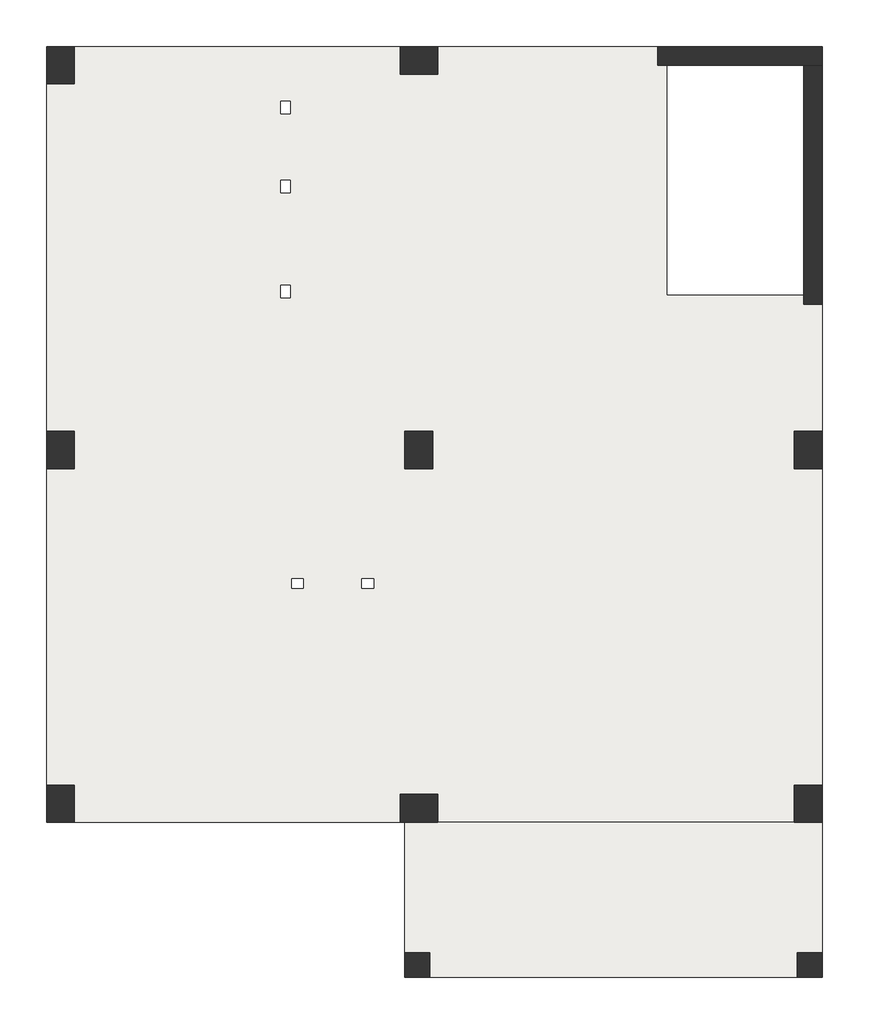
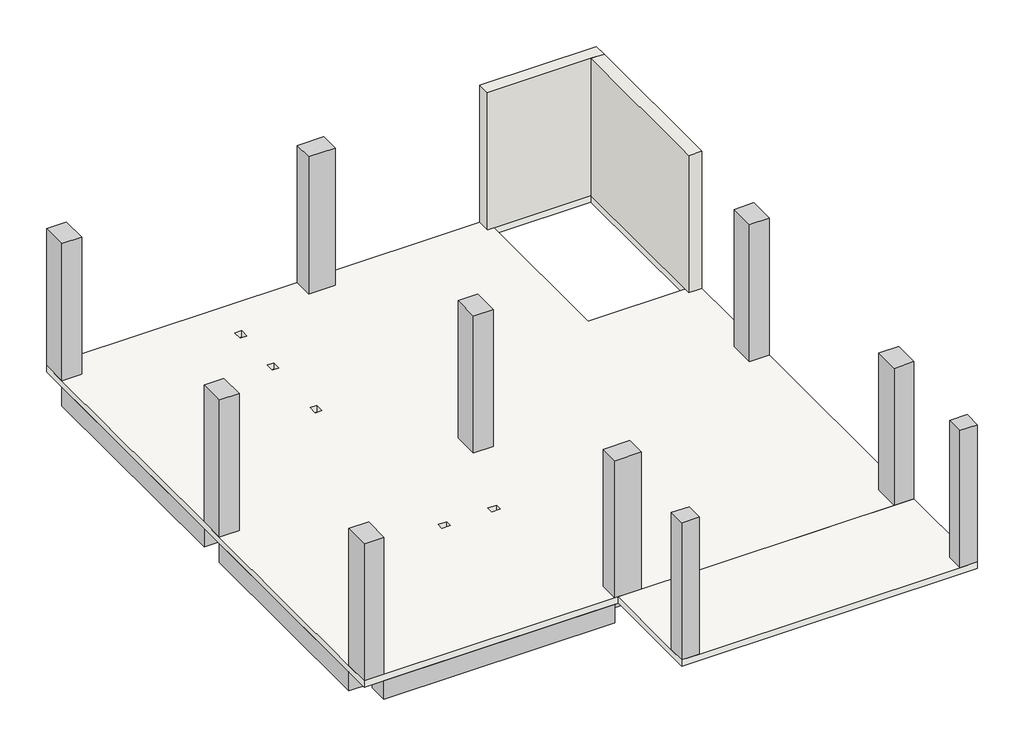
# One storey: 12 beams, 10 columns, 2 slabs, 2 walls.
"""IFC4 building model written with IfcOpenShell, lengths in millimetres."""

from ifc_helpers import new_model, si_unit, frame, origin, place, context, project, spatial, polyline, outline, extrude, faceted_brep, element, save

model = new_model("IFC4")

# Units and contexts
model_context = context("Model", 3, world=origin())
ifc_project = project(units=[si_unit("LENGTHUNIT", "METRE", prefix="MILLI")], contexts=[model_context])

# Site, building, storey
site = spatial("IfcSite", under=ifc_project)
building = spatial("IfcBuilding", under=site)
storey = spatial("IfcBuildingStorey", under=building, Name="01-Birinci Kat", Elevation=97280.0)

# Beams
placement = place(None, origin())
element("IfcBeam", 1, ObjectType="M_Concrete-Rectangular Beam : 45x60cm Kiriş", at=placement, inside=storey, context=model_context, shape_type="SweptSolid", body=[
    extrude(outline(polyline([(5700.0, 14550.0), (450.0, 14550.0), (450.0, 15000.0), (5700.0, 15000.0), (5700.0, 14550.0)])), frame((0.0, 0.0, 96680.0), z_axis=(0.0, 0.0, 1.0), x_axis=(1.0, 0.0, 0.0)), (0.0, 0.0, 1.0), 450.0),
])
element("IfcBeam", 2, ObjectType="M_Concrete-Rectangular Beam : 45x60cm Kiriş", at=placement, inside=storey, context=model_context, shape_type="SweptSolid", body=[
    extrude(outline(polyline([(0.0, 3100.0), (0.0, 8200.0), (450.0, 8200.0), (450.0, 3100.0), (0.0, 3100.0)])), frame((0.0, 0.0, 96680.0), z_axis=(0.0, 0.0, 1.0), x_axis=(1.0, 0.0, 0.0)), (0.0, 0.0, 1.0), 450.0),
])
element("IfcBeam", 3, ObjectType="M_Concrete-Rectangular Beam : 45x60cm Kiriş", at=placement, inside=storey, context=model_context, shape_type="SweptSolid", body=[
    extrude(outline(polyline([(5700.0, 2500.0), (450.0, 2500.0), (450.0, 2950.0), (5700.0, 2950.0), (5700.0, 2500.0)])), frame((0.0, 0.0, 96680.0), z_axis=(0.0, 0.0, 1.0), x_axis=(1.0, 0.0, 0.0)), (0.0, 0.0, 1.0), 450.0),
])
element("IfcBeam", 4, ObjectType="M_Concrete-Rectangular Beam : 45x60cm Kiriş", at=placement, inside=storey, context=model_context, shape_type="SweptSolid", body=[
    extrude(outline(polyline([(12050.0, 2500.0), (6300.0, 2500.0), (6300.0, 2950.0), (12050.0, 2950.0), (12050.0, 2500.0)])), frame((0.0, 0.0, 96680.0), z_axis=(0.0, 0.0, 1.0), x_axis=(1.0, 0.0, 0.0)), (0.0, 0.0, 1.0), 450.0),
])
element("IfcBeam", 5, ObjectType="M_Concrete-Rectangular Beam : 45x60cm Kiriş", at=placement, inside=storey, context=model_context, shape_type="SweptSolid", body=[
    extrude(outline(polyline([(12500.0, 8200.0), (12500.0, 3100.0), (12050.0, 3100.0), (12050.0, 8200.0), (12500.0, 8200.0)])), frame((0.0, 0.0, 96680.0), z_axis=(0.0, 0.0, 1.0), x_axis=(1.0, 0.0, 0.0)), (0.0, 0.0, 1.0), 450.0),
])
element("IfcBeam", 6, ObjectType="M_Concrete-Rectangular Beam : 45x60cm Kiriş", at=placement, inside=storey, context=model_context, shape_type="SweptSolid", body=[
    extrude(outline(polyline([(0.0, 8800.0), (0.0, 14400.0), (450.0, 14400.0), (450.0, 8800.0), (0.0, 8800.0)])), frame((0.0, 0.0, 96680.0), z_axis=(0.0, 0.0, 1.0), x_axis=(1.0, 0.0, 0.0)), (0.0, 0.0, 1.0), 450.0),
])
element("IfcBeam", 7, ObjectType="M_Concrete-Rectangular Beam : 45x60cm Kiriş", at=placement, inside=storey, context=model_context, shape_type="SweptSolid", body=[
    extrude(outline(polyline([(5775.0, 8800.0), (5775.0, 14550.0), (6225.0, 14550.0), (6225.0, 8800.0), (5775.0, 8800.0)])), frame((0.0, 0.0, 96680.0), z_axis=(0.0, 0.0, 1.0), x_axis=(1.0, 0.0, 0.0)), (0.0, 0.0, 1.0), 450.0),
])
element("IfcBeam", 8, ObjectType="M_Concrete-Rectangular Beam : 30x60cm Kiriş", at=placement, inside=storey, context=model_context, shape_type="SweptSolid", body=[
    extrude(outline(polyline([(9850.0, 15000.0), (9850.0, 14700.0), (6300.0, 14700.0), (6300.0, 15000.0), (9850.0, 15000.0)])), frame((0.0, 0.0, 96680.0), z_axis=(0.0, 0.0, 1.0), x_axis=(1.0, 0.0, 0.0)), (0.0, 0.0, 1.0), 450.0),
])
element("IfcBeam", 9, ObjectType="M_Concrete-Rectangular Beam : 30x60cm Kiriş", at=placement, inside=storey, context=model_context, shape_type="SweptSolid", body=[
    extrude(outline(polyline([(12200.0, 10850.0), (12500.0, 10850.0), (12500.0, 8800.0), (12200.0, 8800.0), (12200.0, 10850.0)])), frame((0.0, 0.0, 96680.0), z_axis=(0.0, 0.0, 1.0), x_axis=(1.0, 0.0, 0.0)), (0.0, 0.0, 1.0), 450.0),
])
element("IfcBeam", 10, ObjectType="M_Concrete-Rectangular Beam : 45x60cm Kiriş", at=placement, inside=storey, context=model_context, shape_type="SweptSolid", body=[
    extrude(outline(polyline([(5775.0, 2950.0), (5775.0, 8200.0), (6225.0, 8200.0), (6225.0, 2950.0), (5775.0, 2950.0)])), frame((0.0, 0.0, 96680.0), z_axis=(0.0, 0.0, 1.0), x_axis=(1.0, 0.0, 0.0)), (0.0, 0.0, 1.0), 450.0),
])
element("IfcBeam", 11, ObjectType="M_Concrete-Rectangular Beam : 45x60cm Kiriş", at=placement, inside=storey, context=model_context, shape_type="SweptSolid", body=[
    extrude(outline(polyline([(5775.0, 8275.0), (450.0, 8275.0), (450.0, 8725.0), (5775.0, 8725.0), (5775.0, 8275.0)])), frame((0.0, 0.0, 96680.0), z_axis=(0.0, 0.0, 1.0), x_axis=(1.0, 0.0, 0.0)), (0.0, 0.0, 1.0), 450.0),
])
element("IfcBeam", 12, ObjectType="M_Concrete-Rectangular Beam : 45x60cm Kiriş", at=placement, inside=storey, context=model_context, shape_type="SweptSolid", body=[
    extrude(outline(polyline([(12050.0, 8275.0), (6225.0, 8275.0), (6225.0, 8725.0), (12050.0, 8725.0), (12050.0, 8275.0)])), frame((0.0, 0.0, 96680.0), z_axis=(0.0, 0.0, 1.0), x_axis=(1.0, 0.0, 0.0)), (0.0, 0.0, 1.0), 450.0),
])

# Columns
element("IfcColumn", 13, ObjectType="M_Concrete-Rectangular-Column : 45x60cm Kolon", at=placement, inside=storey, context=model_context, shape_type="SweptSolid", body=[
    extrude(outline(polyline([(450.0, 15000.0), (450.0, 14400.0), (0.0, 14400.0), (0.0, 15000.0), (450.0, 15000.0)])), frame((0.0, 0.0, 97280.0), z_axis=(0.0, 0.0, 1.0), x_axis=(1.0, 0.0, 0.0)), (0.0, 0.0, 1.0), 3300.0),
])
element("IfcColumn", 14, ObjectType="M_Concrete-Rectangular-Column : 45x60cm Kolon", at=placement, inside=storey, context=model_context, shape_type="SweptSolid", body=[
    extrude(outline(polyline([(450.0, 8800.0), (450.0, 8200.0), (0.0, 8200.0), (0.0, 8800.0), (450.0, 8800.0)])), frame((0.0, 0.0, 97280.0), z_axis=(0.0, 0.0, 1.0), x_axis=(1.0, 0.0, 0.0)), (0.0, 0.0, 1.0), 3300.0),
])
element("IfcColumn", 15, ObjectType="M_Concrete-Rectangular-Column : 45x60cm Kolon", at=placement, inside=storey, context=model_context, shape_type="SweptSolid", body=[
    extrude(outline(polyline([(450.0, 3100.0), (450.0, 2500.0), (0.0, 2500.0), (0.0, 3100.0), (450.0, 3100.0)])), frame((0.0, 0.0, 97280.0), z_axis=(0.0, 0.0, 1.0), x_axis=(1.0, 0.0, 0.0)), (0.0, 0.0, 1.0), 3300.0),
])
element("IfcColumn", 16, ObjectType="M_Concrete-Rectangular-Column : 45x60cm Kolon", at=placement, inside=storey, context=model_context, shape_type="SweptSolid", body=[
    extrude(outline(polyline([(6225.0, 8800.0), (6225.0, 8200.0), (5775.0, 8200.0), (5775.0, 8800.0), (6225.0, 8800.0)])), frame((0.0, 0.0, 97280.0), z_axis=(0.0, 0.0, 1.0), x_axis=(1.0, 0.0, 0.0)), (0.0, 0.0, 1.0), 3300.0),
])
element("IfcColumn", 17, ObjectType="M_Concrete-Rectangular-Column : 45x60cm Kolon", at=placement, inside=storey, context=model_context, shape_type="SweptSolid", body=[
    extrude(outline(polyline([(12500.0, 8800.0), (12500.0, 8200.0), (12050.0, 8200.0), (12050.0, 8800.0), (12500.0, 8800.0)])), frame((0.0, 0.0, 97280.0), z_axis=(0.0, 0.0, 1.0), x_axis=(1.0, 0.0, 0.0)), (0.0, 0.0, 1.0), 3300.0),
])
element("IfcColumn", 18, ObjectType="M_Concrete-Rectangular-Column : 45x60cm Kolon", at=placement, inside=storey, context=model_context, shape_type="SweptSolid", body=[
    extrude(outline(polyline([(12500.0, 3100.0), (12500.0, 2500.0), (12050.0, 2500.0), (12050.0, 3100.0), (12500.0, 3100.0)])), frame((0.0, 0.0, 97280.0), z_axis=(0.0, 0.0, 1.0), x_axis=(1.0, 0.0, 0.0)), (0.0, 0.0, 1.0), 3300.0),
])
element("IfcColumn", 19, ObjectType="M_Concrete-Rectangular-Column : 45x60cm Kolon", at=placement, inside=storey, context=model_context, shape_type="SweptSolid", body=[
    extrude(outline(polyline([(5700.0, 15000.0), (6300.0, 15000.0), (6300.0, 14550.0), (5700.0, 14550.0), (5700.0, 15000.0)])), frame((0.0, 0.0, 97280.0), z_axis=(0.0, 0.0, 1.0), x_axis=(1.0, 0.0, 0.0)), (0.0, 0.0, 1.0), 3300.0),
])
element("IfcColumn", 20, ObjectType="M_Concrete-Rectangular-Column : 40x40cm Kolon", at=placement, inside=storey, context=model_context, shape_type="SweptSolid", body=[
    extrude(outline(polyline([(6175.0, 400.0), (6175.0, 0.0), (5775.0, 0.0), (5775.0, 400.0), (6175.0, 400.0)])), frame((0.0, 0.0, 97280.0), z_axis=(0.0, 0.0, 1.0), x_axis=(1.0, 0.0, 0.0)), (0.0, 0.0, 1.0), 3300.0),
])
element("IfcColumn", 21, ObjectType="M_Concrete-Rectangular-Column : 45x60cm Kolon", at=placement, inside=storey, context=model_context, shape_type="SweptSolid", body=[
    extrude(outline(polyline([(5700.0, 2950.0), (6300.0, 2950.0), (6300.0, 2500.0), (5700.0, 2500.0), (5700.0, 2950.0)])), frame((0.0, 0.0, 97280.0), z_axis=(0.0, 0.0, 1.0), x_axis=(1.0, 0.0, 0.0)), (0.0, 0.0, 1.0), 3300.0),
])
element("IfcColumn", 22, ObjectType="M_Concrete-Rectangular-Column : 40x40cm Kolon", at=placement, inside=storey, context=model_context, shape_type="SweptSolid", body=[
    extrude(outline(polyline([(12500.0, 400.0), (12500.0, 0.0), (12100.0, 0.0), (12100.0, 400.0), (12500.0, 400.0)])), frame((0.0, 0.0, 97280.0), z_axis=(0.0, 0.0, 1.0), x_axis=(1.0, 0.0, 0.0)), (0.0, 0.0, 1.0), 3300.0),
])

# Slabs
element("IfcSlab", 23, ObjectType="15 cm döşeme", at=placement, inside=storey, context=model_context, shape_type="Brep", body=[
    faceted_brep([(12500.0, 15000.0, 97130.0), (12500.0, 10850.0, 97130.0), (12500.0, 8800.0, 97130.0), (12500.0, 8200.0, 97130.0), (12500.0, 3100.0, 97130.0), (12500.0, 2500.0, 97130.0), (12050.0, 2500.0, 97130.0), (6300.0, 2500.0, 97130.0), (5700.0, 2500.0, 97130.0), (450.0, 2500.0, 97130.0), (0.0, 2500.0, 97130.0), (0.0, 3100.0, 97130.0), (0.0, 8200.0, 97130.0), (0.0, 8800.0, 97130.0), (0.0, 14400.0, 97130.0), (0.0, 15000.0, 97130.0), (450.0, 15000.0, 97130.0), (5700.0, 15000.0, 97130.0), (6300.0, 15000.0, 97130.0), (9850.0, 15000.0, 97130.0), (12200.0, 11000.0, 97130.0), (12200.0, 14700.0, 97130.0), (10000.0, 14700.0, 97130.0), (10000.0, 11000.0, 97130.0), (5078.0485114, 6275.0, 97130.0), (5275.0, 6275.0, 97130.0), (5275.0, 6420.7099889, 97130.0), (5078.0485114, 6420.7099889, 97130.0), (4140.0485128, 6275.0, 97130.0), (4140.0485128, 6420.7099889, 97130.0), (3949.7459943, 6420.7099889, 97130.0), (3949.7459943, 6275.0, 97130.0), (3925.0, 11154.975, 97130.0), (3775.0, 11154.975, 97130.0), (3775.0, 10954.975, 97130.0), (3925.0, 10954.975, 97130.0), (3925.0, 12846.5789726, 97130.0), (3775.0, 12846.5789726, 97130.0), (3775.0, 12646.5789726, 97130.0), (3925.0, 12646.5789726, 97130.0), (3925.0, 14120.0, 97130.0), (3775.0, 14120.0, 97130.0), (3775.0, 13920.0, 97130.0), (3925.0, 13920.0, 97130.0), (12500.0, 15000.0, 97280.0), (6300.0, 15000.0, 97280.0), (5700.0, 15000.0, 97280.0), (450.0, 15000.0, 97280.0), (0.0, 15000.0, 97280.0), (0.0, 14400.0, 97280.0), (0.0, 8800.0, 97280.0), (0.0, 8200.0, 97280.0), (0.0, 3100.0, 97280.0), (0.0, 2500.0, 97280.0), (450.0, 2500.0, 97280.0), (5700.0, 2500.0, 97280.0), (6300.0, 2500.0, 97280.0), (12050.0, 2500.0, 97280.0), (12500.0, 2500.0, 97280.0), (12500.0, 3100.0, 97280.0), (12500.0, 8200.0, 97280.0), (12500.0, 8800.0, 97280.0), (12200.0, 11000.0, 97280.0), (10000.0, 11000.0, 97280.0), (10000.0, 14700.0, 97280.0), (12200.0, 14700.0, 97280.0), (5078.0485114, 6275.0, 97280.0), (5078.0485114, 6420.7099889, 97280.0), (5275.0, 6420.7099889, 97280.0), (5275.0, 6275.0, 97280.0), (4140.0485128, 6275.0, 97280.0), (3949.7459943, 6275.0, 97280.0), (3949.7459943, 6420.7099889, 97280.0), (4140.0485128, 6420.7099889, 97280.0), (3925.0, 11154.975, 97280.0), (3925.0, 10954.975, 97280.0), (3775.0, 10954.975, 97280.0), (3775.0, 11154.975, 97280.0), (3925.0, 12846.5789726, 97280.0), (3925.0, 12646.5789726, 97280.0), (3775.0, 12646.5789726, 97280.0), (3775.0, 12846.5789726, 97280.0), (3925.0, 14120.0, 97280.0), (3925.0, 13920.0, 97280.0), (3775.0, 13920.0, 97280.0), (3775.0, 14120.0, 97280.0)], [[[0, 1, 2, 3, 4, 5, 6, 7, 8, 9, 10, 11, 12, 13, 14, 15, 16, 17, 18, 19], [20, 21, 22, 23], [24, 25, 26, 27], [28, 29, 30, 31], [32, 33, 34, 35], [36, 37, 38, 39], [40, 41, 42, 43]], [[44, 45, 46, 47, 48, 49, 50, 51, 52, 53, 54, 55, 56, 57, 58, 59, 60, 61], [62, 63, 64, 65], [66, 67, 68, 69], [70, 71, 72, 73], [74, 75, 76, 77], [78, 79, 80, 81], [82, 83, 84, 85]], [[5, 4, 3, 2, 1, 0, 44, 61, 60, 59, 58]], [[10, 9, 8, 7, 6, 5, 58, 57, 56, 55, 54, 53]], [[15, 14, 13, 12, 11, 10, 53, 52, 51, 50, 49, 48]], [[0, 19, 18, 17, 16, 15, 48, 47, 46, 45, 44]], [[21, 20, 62, 65]], [[22, 21, 65, 64]], [[23, 22, 64, 63]], [[20, 23, 63, 62]], [[25, 24, 66, 69]], [[26, 25, 69, 68]], [[27, 26, 68, 67]], [[24, 27, 67, 66]], [[29, 28, 70, 73]], [[30, 29, 73, 72]], [[31, 30, 72, 71]], [[28, 31, 71, 70]], [[33, 32, 74, 77]], [[34, 33, 77, 76]], [[35, 34, 76, 75]], [[32, 35, 75, 74]], [[37, 36, 78, 81]], [[38, 37, 81, 80]], [[39, 38, 80, 79]], [[36, 39, 79, 78]], [[41, 40, 82, 85]], [[42, 41, 85, 84]], [[43, 42, 84, 83]], [[40, 43, 83, 82]]]),
])
element("IfcSlab", 24, ObjectType="15 cm döşeme", at=placement, inside=storey, context=model_context, shape_type="Brep", body=[
    faceted_brep([(12500.0, 2500.0, 97130.0), (12500.0, 450.0, 97130.0), (12500.0, 0.0, 97130.0), (12050.0, 0.0, 97130.0), (6225.0, 0.0, 97130.0), (5775.0, 0.0, 97130.0), (5775.0, 450.0, 97130.0), (5775.0, 2500.0, 97130.0), (12500.0, 2500.0, 97280.0), (5775.0, 2500.0, 97280.0), (5775.0, 400.0, 97280.0), (5775.0, 0.0, 97280.0), (6175.0, 0.0, 97280.0), (12100.0, 0.0, 97280.0), (12500.0, 0.0, 97280.0), (12500.0, 400.0, 97280.0)], [[[0, 1, 2, 3, 4, 5, 6, 7]], [[8, 9, 10, 11, 12, 13, 14, 15]], [[2, 1, 0, 8, 15, 14]], [[5, 4, 3, 2, 14, 13, 12, 11]], [[7, 6, 5, 11, 10, 9]], [[0, 7, 9, 8]]]),
])

# Walls
element("IfcWall", 25, ObjectType="30cm Perde Duvar", at=placement, inside=storey, context=model_context, shape_type="Brep", body=[
    faceted_brep([(9850.0, 14700.0, 97280.0), (12200.0, 14700.0, 97280.0), (12500.0, 14700.0, 97280.0), (12500.0, 14700.0, 100580.0), (12200.0, 14700.0, 100580.0), (9850.0, 14700.0, 100580.0), (9850.0, 14700.0, 100180.0), (9850.0, 15000.0, 97280.0), (9850.0, 15000.0, 100180.0), (9850.0, 15000.0, 100580.0), (12500.0, 15000.0, 100580.0), (12500.0, 15000.0, 97280.0)], [[[0, 1, 2, 3, 4, 5, 6]], [[7, 8, 9, 10, 11]], [[2, 1, 0, 7, 11]], [[0, 6, 5, 9, 8, 7]], [[3, 2, 11, 10]], [[5, 4, 3, 10, 9]]]),
])
element("IfcWall", 26, ObjectType="30cm Perde Duvar", at=placement, inside=storey, context=model_context, shape_type="Brep", body=[
    faceted_brep([(12200.0, 14700.0, 97280.0), (12200.0, 10850.0, 97280.0), (12200.0, 10850.0, 100180.0), (12200.0, 10850.0, 100580.0), (12200.0, 14700.0, 100580.0), (12500.0, 14700.0, 97280.0), (12500.0, 14700.0, 100580.0), (12500.0, 10850.0, 100580.0), (12500.0, 10850.0, 100180.0), (12500.0, 10850.0, 97280.0)], [[[0, 1, 2, 3, 4]], [[5, 6, 7, 8, 9]], [[1, 0, 5, 9]], [[3, 2, 1, 9, 8, 7]], [[0, 4, 6, 5]], [[4, 3, 7, 6]]]),
])

save(model, "model.ifc")

# Revit data of these elements
# Type "M_Concrete-Rectangular Beam : 45x60cm Kiriş"
#   Length [instance default] = 152.40 cm
#   b = 45.00 cm
#   h = 60.00 cm
#   Structural Material [instance default] = Concrete, Cast-in-Place gray
#   Assembly Code = ""
# Type "M_Concrete-Rectangular Beam : 30x60cm Kiriş"
#   Length [instance default] = 152.40 cm
#   b = 30.00 cm
#   h = 60.00 cm
#   Structural Material [instance default] = Concrete, Cast-in-Place gray
#   Assembly Code = ""
# Type "M_Concrete-Rectangular-Column : 45x60cm Kolon"
#   b = 45.00 cm
#   h = 60.00 cm
#   Structural Material [instance default] = Concrete, Cast-in-Place gray
# Type "M_Concrete-Rectangular-Column : 40x40cm Kolon"
#   b = 40.00 cm
#   h = 40.00 cm
#   Structural Material [instance default] = Concrete, Cast-in-Place gray
# Type "15 cm döşeme"
#   Function = 0
#   Layers, outside or top first: 15.00 cm "Concrete, Cast In Situ" (function 1)
# Type "30cm Perde Duvar"
#   Layers, outside or top first: 30.00 cm "Concrete, Cast In Situ" (function 1)
# Elements 1, 2, 3, 4, 5, 6, 7, 10, 11, 12 (IfcBeam, "M_Concrete-Rectangular Beam : 45x60cm Kiriş")
#   Comments = ""
#   Structural Material = Concrete, Cast-in-Place gray
#   Phase Created = New Construction
#   Materials on its faces: "Concrete, Cast-in-Place gray"
# Elements 8, 9 (IfcBeam, "M_Concrete-Rectangular Beam : 30x60cm Kiriş")
#   Comments = ""
#   Structural Material = Concrete, Cast-in-Place gray
#   Phase Created = New Construction
#   Materials on its faces: "Concrete, Cast-in-Place gray"
# Elements 13, 14, 15, 16, 17, 18, 19, 21 (IfcColumn, "M_Concrete-Rectangular-Column : 45x60cm Kolon")
#   Comments = ""
#   Structural Material = Concrete, Cast-in-Place gray
#   Phase Created = New Construction
#   Materials on its faces: "Concrete, Cast-in-Place gray"
# Elements 20, 22 (IfcColumn, "M_Concrete-Rectangular-Column : 40x40cm Kolon")
#   Comments = ""
#   Structural Material = Concrete, Cast-in-Place gray
#   Phase Created = New Construction
#   Materials on its faces: "Concrete, Cast-in-Place gray"
# Elements 23, 24 (IfcSlab, "15 cm döşeme")
#   Height Offset From Level = 0.00 cm
#   built-in parameter 1001954 = 1
#   Phase Created = New Construction
#   Materials on its faces: "Concrete, Cast In Situ"
# Elements 25, 26 (IfcWall, "30cm Perde Duvar")
#   Comments = ""
#   Top Offset = 0.00 cm
#   Base Offset = 0.00 cm
#   wall height = 330.00 cm
#   Phase Created = New Construction
#   Base Constraint = 01-Birinci Kat
#   Top Constraint = 02-Çatı Katı
#   Materials on its faces: "Concrete, Cast In Situ"
# Materials
#   "Concrete, Cast-in-Place gray": class "Concrete", colour RGB 192 192 192, transparency 0, Description = "Cast-in-place concrete", Cost = 0
#   "Concrete, Cast In Situ": class "Concrete", colour RGB 192 192 192, transparency 0, Description = "physical material", Cost = 0
